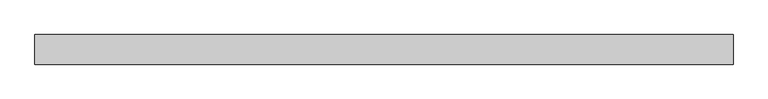
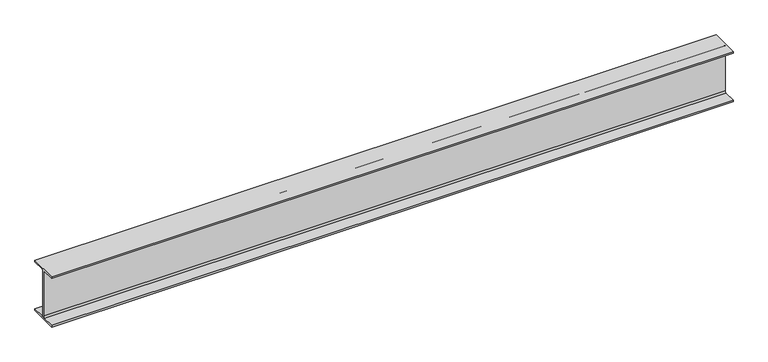
"""IFC4 building model written with IfcOpenShell, lengths in millimetres: beam geometry, Old_Steel Beam_H-KSD3502 : H_SB_ASB_H-200×200x8x12."""

import ifcopenshell
import ifcopenshell.guid

model = None  # the IFC model being written
_history = None  # IfcOwnerHistory: only IFC2X3 demands one
_inside = {}  # id of a spatial element -> (the spatial element, [elements in it])
_under = {}  # id of a project, library or spatial element -> (it, [spatial elements below it])
_declared = {}  # id of a project -> (the project, [libraries it declares])
_typed = {}  # id of a type object -> (the type object, [elements of that type])
_made_of = {}  # id of a material, layer set ... -> (it, [elements and type objects made of it])


def new_model(schema):
    """Start an empty IFC model of exactly this schema.

    Asked for "IFC4X3", IfcOpenShell would pick the latest addendum, in which some entities
    have other attributes; the version numbers below select the first issue.
    IFC2X3 requires an IfcOwnerHistory on every rooted entity: one is made here for all.
    """
    global model, _history
    if schema == "IFC4X3":
        model = ifcopenshell.file(schema_version=(4, 3, 0, 0))
    else:
        model = ifcopenshell.file(schema=schema)
    _inside.clear()
    _under.clear()
    _declared.clear()
    _typed.clear()
    _made_of.clear()
    _history = None
    if model.schema == "IFC2X3":
        org = make("IfcOrganization", Name="unknown")
        user = make(
            "IfcPersonAndOrganization",
            ThePerson=make("IfcPerson", FamilyName="unknown"),
            TheOrganization=org,
        )
        app = make(
            "IfcApplication",
            ApplicationDeveloper=org,
            Version="unknown",
            ApplicationFullName="unknown",
            ApplicationIdentifier="unknown",
        )
        _history = make(
            "IfcOwnerHistory",
            OwningUser=user,
            OwningApplication=app,
            ChangeAction="ADDED",
            CreationDate=0,
        )
    return model


def make(cls, **values):
    """One entity of the class cls with the attributes given. An attribute that is None is left unset."""
    return model.create_entity(
        cls, **{name: value for name, value in values.items() if value is not None}
    )


def rooted(cls, **values):
    """An entity with a GlobalId (a new one), such as an element, a storey or a relation."""
    return make(cls, GlobalId=ifcopenshell.guid.new(), OwnerHistory=_history, **values)


def si_unit(unit_type, name, prefix=None):
    """IfcSIUnit, for example si_unit("LENGTHUNIT", "METRE", prefix="MILLI")."""
    return make("IfcSIUnit", UnitType=unit_type, Prefix=prefix, Name=name)


def assignment(units):
    """IfcUnitAssignment: the units of a project."""
    return None if units is None else make("IfcUnitAssignment", Units=units)


def point(xyz):
    """IfcCartesianPoint."""
    return None if xyz is None else make("IfcCartesianPoint", Coordinates=xyz)


def direction(xyz):
    """IfcDirection."""
    return None if xyz is None else make("IfcDirection", DirectionRatios=xyz)


def frame(location, z_axis=None, x_axis=None):
    """IfcAxis2Placement3D, a coordinate frame: its origin and axes. An axis left out is left unset."""
    return make(
        "IfcAxis2Placement3D",
        Location=point(location),
        Axis=direction(z_axis),
        RefDirection=direction(x_axis),
    )


def frame_2d(location, x_axis=None):
    """IfcAxis2Placement2D, a coordinate frame in the plane: its origin and x axis."""
    return make(
        "IfcAxis2Placement2D", Location=point(location), RefDirection=direction(x_axis)
    )


def origin():
    """The frame at (0, 0, 0) with its axes left unset."""
    return frame((0.0, 0.0, 0.0))


def place(relative_to, where):
    """IfcLocalPlacement: puts the frame where relative to a parent placement (None: the world)."""
    return make(
        "IfcLocalPlacement", PlacementRelTo=relative_to, RelativePlacement=where
    )


def context(
    kind, dimensions, precision=None, world=None, true_north=None, identifier=None
):
    """IfcGeometricRepresentationContext, for example the 3D "Model" context."""
    return make(
        "IfcGeometricRepresentationContext",
        ContextIdentifier=identifier,
        ContextType=kind,
        CoordinateSpaceDimension=dimensions,
        Precision=precision,
        WorldCoordinateSystem=world,
        TrueNorth=true_north,
    )


def project(units=None, contexts=None):
    """IfcProject with its units and contexts."""
    return rooted(
        "IfcProject",
        Name="project",
        RepresentationContexts=contexts,
        UnitsInContext=assignment(units),
    )


def spatial(cls, under=None, at=None, **own):
    """A site, building, storey or space (cls), placed at a placement, below another one or the project."""
    s = rooted(cls, ObjectPlacement=at, **own)
    if under is not None:
        _under.setdefault(under.id(), (under, []))[1].append(s)
    return s


def polyline(points):
    """IfcPolyline through the points."""
    return make("IfcPolyline", Points=[point(p) for p in points])


def circle_curve(where, radius):
    """IfcCircle in the frame where."""
    return make("IfcCircle", Position=where, Radius=radius)


def trimmed(basis, trim1, trim2, sense, master):
    """IfcTrimmedCurve: the piece of a basis curve between two trims."""
    return make(
        "IfcTrimmedCurve",
        BasisCurve=basis,
        Trim1=trim1,
        Trim2=trim2,
        SenseAgreement=sense,
        MasterRepresentation=master,
    )


def segment(curve, same_sense, transition):
    """IfcCompositeCurveSegment."""
    return make(
        "IfcCompositeCurveSegment",
        Transition=transition,
        SameSense=same_sense,
        ParentCurve=curve,
    )


def composite_curve(segments, self_intersect=None):
    """IfcCompositeCurve: segments joined end to end."""
    return make("IfcCompositeCurve", Segments=segments, SelfIntersect=self_intersect)


def outline(outer, holes=None, kind="AREA"):
    """IfcArbitraryClosedProfileDef: a profile drawn as a closed curve; with holes, ...WithVoids."""
    if holes is None:
        return make("IfcArbitraryClosedProfileDef", ProfileType=kind, OuterCurve=outer)
    return make(
        "IfcArbitraryProfileDefWithVoids",
        ProfileType=kind,
        OuterCurve=outer,
        InnerCurves=holes,
    )


def extrude(swept, where, along, depth):
    """IfcExtrudedAreaSolid: the profile swept, set in the frame where, extruded along a direction by depth."""
    return make(
        "IfcExtrudedAreaSolid",
        SweptArea=swept,
        Position=where,
        ExtrudedDirection=direction(along),
        Depth=depth,
    )


def shape(context_of_items, identifier, shape_type, items):
    """IfcShapeRepresentation: the items that make up one representation, for example the "Body"."""
    return make(
        "IfcShapeRepresentation",
        ContextOfItems=context_of_items,
        RepresentationIdentifier=identifier,
        RepresentationType=shape_type,
        Items=items,
    )


def source(mapping_origin, context_of_items, identifier, shape_type, items):
    """IfcRepresentationMap: a shape defined once, which mapped items show again and again."""
    return make(
        "IfcRepresentationMap",
        MappingOrigin=mapping_origin,
        MappedRepresentation=shape(context_of_items, identifier, shape_type, items),
    )


def transform(
    local_origin,
    x_axis=None,
    y_axis=None,
    z_axis=None,
    scale=None,
    scale2=None,
    scale3=None,
    uniform=True,
):
    """IfcCartesianTransformationOperator3D, or its non-uniform kind. x_axis, y_axis, z_axis: its Axis1, 2, 3."""
    if uniform:
        return make(
            "IfcCartesianTransformationOperator3D",
            Axis1=direction(x_axis),
            Axis2=direction(y_axis),
            LocalOrigin=point(local_origin),
            Scale=scale,
            Axis3=direction(z_axis),
        )
    return make(
        "IfcCartesianTransformationOperator3DnonUniform",
        Axis1=direction(x_axis),
        Axis2=direction(y_axis),
        LocalOrigin=point(local_origin),
        Scale=scale,
        Axis3=direction(z_axis),
        Scale2=scale2,
        Scale3=scale3,
    )


def mapped(mapping_source, mapping_target):
    """IfcMappedItem: shows the shape of a source again, moved by a transform."""
    return make(
        "IfcMappedItem", MappingSource=mapping_source, MappingTarget=mapping_target
    )


def made_of(thing, what):
    """Note that an element or type object is made of a material, layer set ...; save() writes the relation."""
    if what is not None:
        _made_of.setdefault(what.id(), (what, []))[1].append(thing)
    return thing


def element(
    cls,
    number,
    at=None,
    inside=None,
    cuts=None,
    type_object=None,
    material=None,
    context=None,
    identifier="Body",
    shape_type=None,
    held_by="IfcProductDefinitionShape",
    body=None,
    shapes=None,
    **own,
):
    """One element of the class cls, such as IfcWall. Its Tag is "e" and its number.

    at: its placement. inside: the storey or other place that contains it. cuts: it is an
    opening in that element (IfcRelVoidsElement). A single representation is given by context,
    identifier, shape_type and body (its items); several are given by shapes. held_by: the class
    of the entity that holds the representations. save() writes the other relations.
    """
    e = rooted(cls, Tag="e%d" % number, ObjectPlacement=at, **own)
    if body is not None:
        shapes = [shape(context, identifier, shape_type, body)]
    if shapes is not None:
        e.Representation = make(held_by, Representations=shapes)
    if inside is not None:
        _inside.setdefault(inside.id(), (inside, []))[1].append(e)
    if cuts is not None:
        rooted(
            "IfcRelVoidsElement", RelatingBuildingElement=cuts, RelatedOpeningElement=e
        )
    if type_object is not None:
        _typed.setdefault(type_object.id(), (type_object, []))[1].append(e)
    return made_of(e, material)


def aggregate(whole, parts):
    """IfcRelAggregates: a whole, such as a stair, and the parts it consists of."""
    return rooted("IfcRelAggregates", RelatingObject=whole, RelatedObjects=parts)


def save(model, path):
    """Write the relations noted so far, then the file.

    IfcRelAggregates (storeys below a building ...), IfcRelContainedInSpatialStructure (elements
    in a storey), IfcRelDefinesByType, IfcRelAssociatesMaterial and IfcRelDeclares: one each for
    every whole, place, type object, material and project.
    """
    for whole, parts in _under.values():
        aggregate(whole, parts)
    for where, things in _inside.values():
        rooted(
            "IfcRelContainedInSpatialStructure",
            RelatedElements=things,
            RelatingStructure=where,
        )
    for kind, things in _typed.values():
        rooted("IfcRelDefinesByType", RelatedObjects=things, RelatingType=kind)
    for what, things in _made_of.values():
        rooted("IfcRelAssociatesMaterial", RelatedObjects=things, RelatingMaterial=what)
    for by, libraries in _declared.values():
        rooted("IfcRelDeclares", RelatingContext=by, RelatedDefinitions=libraries)
    model.write(path)


def beam_e3e9dac9(model_context):
    return source(origin(), model_context, "Body", "SweptSolid", [
        extrude(outline(composite_curve([segment(polyline([(82.5, -141.5), (82.5, -151.7), (-82.5, -151.7), (-82.5, -141.5), (-11.9, -141.5)]), True, "CONTINUOUS"), segment(trimmed(circle_curve(frame_2d((-11.9, -132.6)), 8.9), [point((-11.9, -141.5))], [point((-3.0, -132.6))], True, "CARTESIAN"), True, "CONTINUOUS"), segment(polyline([(-3.0, -132.6), (-3.0, 132.6)]), True, "CONTINUOUS"), segment(trimmed(circle_curve(frame_2d((-11.9, 132.6)), 8.9), [point((-3.0, 132.6))], [point((-11.9, 141.5))], True, "CARTESIAN"), True, "CONTINUOUS"), segment(polyline([(-11.9, 141.5), (-82.5, 141.5), (-82.5, 151.7), (82.5, 151.7), (82.5, 141.5), (11.9, 141.5)]), True, "CONTINUOUS"), segment(trimmed(circle_curve(frame_2d((11.9, 132.6)), 8.9), [point((11.9, 141.5))], [point((3.0, 132.6))], True, "CARTESIAN"), True, "CONTINUOUS"), segment(polyline([(3.0, 132.6), (3.0, -132.6)]), True, "CONTINUOUS"), segment(trimmed(circle_curve(frame_2d((11.9, -132.6)), 8.9), [point((3.0, -132.6))], [point((11.9, -141.5))], True, "CARTESIAN"), True, "CONTINUOUS"), segment(polyline([(11.9, -141.5), (82.5, -141.5)]), True, "CONTINUOUS")], self_intersect=False)), frame((-1898.8220866, 0.0, 0.0), z_axis=(1.0, 0.0, 0.0), x_axis=(0.0, 1.0, 0.0)), (0.0, 0.0, 1.0), 3882.4854417),
    ])


if __name__ == "__main__":
    model = new_model("IFC4")
    model_context = context("Model", 3, world=origin())
    ifc_project = project(units=[si_unit("LENGTHUNIT", "METRE", prefix="MILLI")], contexts=[model_context])
    site = spatial("IfcSite", under=ifc_project)
    building = spatial("IfcBuilding", under=site)
    placement = place(None, origin())
    beam_shape = beam_e3e9dac9(model_context)
    element("IfcBeam", 1, ObjectType="Old_Steel Beam_H-KSD3502 : H_SB_ASB_H-200×200x8x12", at=placement, inside=building, context=model_context, shape_type="MappedRepresentation", body=[
        mapped(beam_shape, transform((0.0, 0.0, 0.0), x_axis=(1.0, 0.0, 0.0), y_axis=(0.0, 1.0, 0.0), z_axis=(0.0, 0.0, 1.0))),
    ])
    save(model, "model.ifc")

# Revit data of these elements
# Type "Old_Steel Beam_H-KSD3502 : H_SB_ASB_H-200×200x8x12"
#   Width = 20.0 cm
#   Web Thickness = 0.8 cm
#   Web Fillet = 1.3 cm
#   Warping Constant = 141376.0 cm⁶
#   Torsional Moment of Inertia = 26.2485 cm⁴
#   Torsional Modulus = 1.0 cm³
#   Section Area = 63.53 cm²
#   Plastic Modulus weak axis = 244.0 cm³
#   Plastic Modulus strong axis = 525.0 cm³
#   Perimeter = 1.16 m²/m
#   Nominal Weight = 49.90 kgf/m
#   Moment of Inertia weak axis = 1600.00 cm⁴
#   Moment of Inertia strong axis = 4720.00 cm⁴
#   Height = 20.0 cm
#   Flange Thickness = 1.2 cm
#   Elastic Modulus weak axis = 160.0 cm³
#   Elastic Modulus strong axis = 472.0 cm³
#   Centroid Vertical = 10.0 cm
#   Centroid Horizontal = 10.0 cm
#   Length [instance default] = 1.5240 m
#   Structural Material [instance default] = Steel, 45-345
#   Assembly Code = ""
# Element 1 (IfcBeam, "Old_Steel Beam_H-KSD3502 : H_SB_ASB_H-200×200x8x12")
#   Structural Material = none
# Materials
#   "Steel, 45-345": class "Metal", colour RGB 189 187 185, transparency 0, Description = "Steel 345 MPa", Cost = 0
